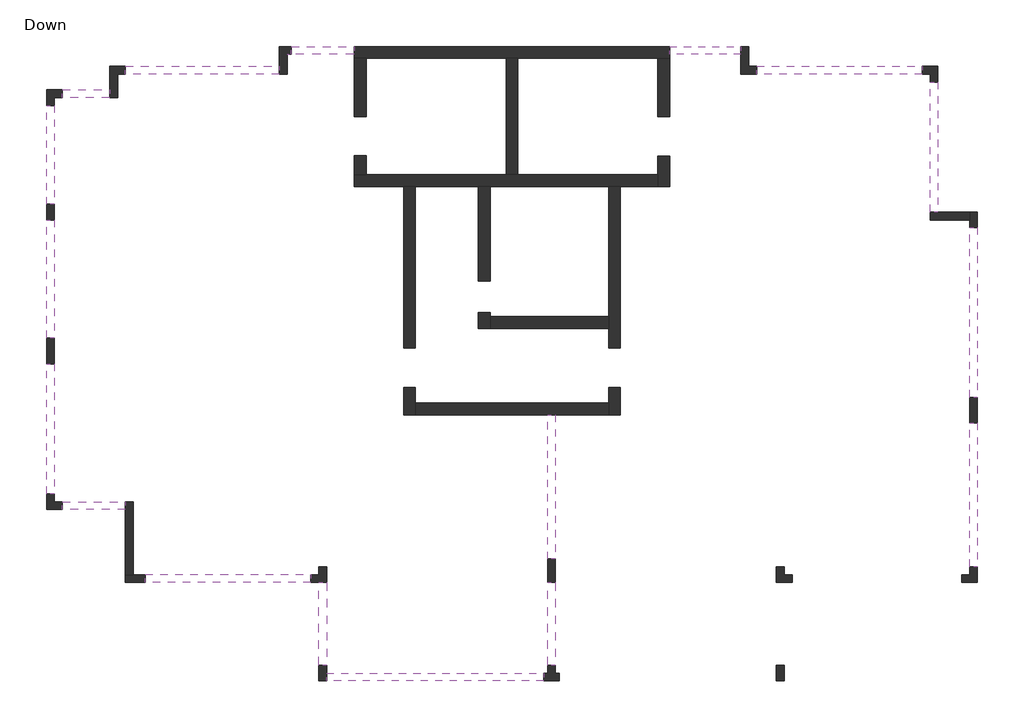
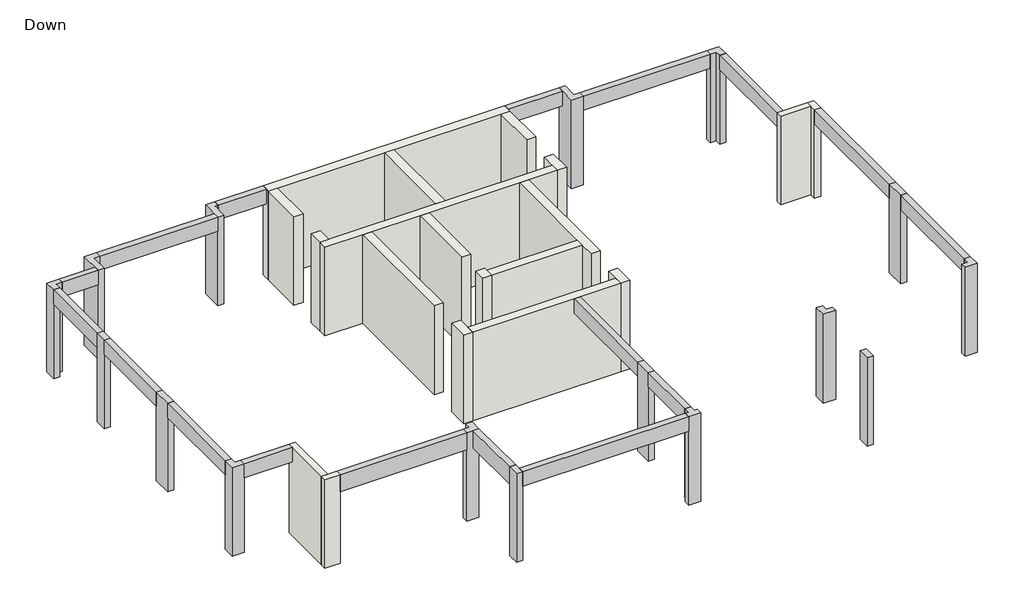
# One storey: 19 walls, 17 beams, 16 columns.
# Revit data of these elements (continued)
# Element 39 (IfcWall, "30") (continued)
#   SOFiSTiK_AMG_Scheduled = yes
#   SOFiSTiK_AMG_Adjusted = yes
#   Phase Created = New Construction
#   Base Constraint = Down
#   Top Constraint = Typical Floor
#   Materials on its faces: "Concrete"
# Element 40 (IfcWall, "30")
#   Comments = ""
#   Mark = "W7"
#   SOFiSTiK_EdgeZones = "W7"
#   SOFiSTiK_AMG_Comments = ""
#   Top Offset = 0 cm
#   Base Offset = 0 cm
#   wall height = 310 cm
#   SOFiSTiK_AMG_Scheduled = yes
#   SOFiSTiK_AMG_Adjusted = yes
#   Phase Created = New Construction
#   Base Constraint = Down
#   Top Constraint = Typical Floor
#   Materials on its faces: "Concrete"
# Element 41 (IfcWall, "30")
#   Comments = ""
#   Mark = "W8"
#   SOFiSTiK_EdgeZones = "W8"
#   SOFiSTiK_AMG_Comments = ""
#   Top Offset = 0 cm
#   Base Offset = 0 cm
#   wall height = 310 cm
#   SOFiSTiK_AMG_Scheduled = yes
#   SOFiSTiK_AMG_Adjusted = yes
#   Phase Created = New Construction
#   Base Constraint = Down
#   Top Constraint = Typical Floor
#   Materials on its faces: "Concrete"
# Element 42 (IfcWall, "30")
#   Comments = ""
#   Mark = "W9"
#   SOFiSTiK_EdgeZones = "W9"
#   SOFiSTiK_AMG_Comments = ""
#   Top Offset = 0 cm
#   Base Offset = 0 cm
#   wall height = 310 cm
#   SOFiSTiK_AMG_Scheduled = yes
#   SOFiSTiK_AMG_Adjusted = yes
#   Phase Created = New Construction
#   Base Constraint = Down
#   Top Constraint = Typical Floor
#   Materials on its faces: "Concrete"
# Element 43 (IfcWall, "30")
#   Comments = ""
#   Mark = "W10"
#   SOFiSTiK_EdgeZones = "W10"
#   SOFiSTiK_AMG_Comments = ""
#   Top Offset = 0 cm
#   Base Offset = 0 cm
#   wall height = 310 cm
#   SOFiSTiK_AMG_Scheduled = yes
#   SOFiSTiK_AMG_Adjusted = yes
#   Phase Created = New Construction
#   Base Constraint = Down
#   Top Constraint = Typical Floor
#   Materials on its faces: "Concrete"
# Element 44 (IfcWall, "30")
#   Comments = ""
#   Mark = "W11"
#   SOFiSTiK_EdgeZones = "W11"
#   SOFiSTiK_AMG_Comments = ""
#   Top Offset = 0 cm
#   Base Offset = 0 cm
#   wall height = 310 cm
#   SOFiSTiK_AMG_Scheduled = yes
#   SOFiSTiK_AMG_Adjusted = yes
#   Phase Created = New Construction
#   Base Constraint = Down
#   Top Constraint = Typical Floor
#   Materials on its faces: "Concrete"
# Element 45 (IfcWall, "30")
#   Comments = ""
#   Mark = "W12"
#   SOFiSTiK_EdgeZones = "W12"
#   SOFiSTiK_AMG_Comments = ""
#   Top Offset = 0 cm
#   Base Offset = 0 cm
#   wall height = 310 cm
#   SOFiSTiK_AMG_Scheduled = yes
#   SOFiSTiK_AMG_Adjusted = yes
#   Phase Created = New Construction
#   Base Constraint = Down
#   Top Constraint = Typical Floor
#   Materials on its faces: "Concrete"
# Element 46 (IfcWall, "30")
#   Comments = ""
#   Mark = "W13"
#   SOFiSTiK_EdgeZones = "W13"
#   SOFiSTiK_AMG_Comments = ""
#   Top Offset = 0 cm
#   Base Offset = 0 cm
#   wall height = 310 cm
#   SOFiSTiK_AMG_Scheduled = yes
#   SOFiSTiK_AMG_Adjusted = yes
#   Phase Created = New Construction
#   Base Constraint = Down
#   Top Constraint = Typical Floor
#   Materials on its faces: "Concrete"
# Element 47 (IfcWall, "30")
#   Comments = ""
#   Mark = "W14"
#   SOFiSTiK_EdgeZones = "W14"
#   SOFiSTiK_AMG_Comments = ""
#   Top Offset = 0 cm
#   Base Offset = 0 cm
#   wall height = 310 cm
#   SOFiSTiK_AMG_Scheduled = yes
#   SOFiSTiK_AMG_Adjusted = yes
#   Phase Created = New Construction
#   Base Constraint = Down
#   Top Constraint = Typical Floor
#   Materials on its faces: "Concrete"
# Element 48 (IfcWall, "30")
#   Comments = ""
#   Mark = "W15"
#   SOFiSTiK_EdgeZones = "W15"
#   SOFiSTiK_AMG_Comments = ""
#   Top Offset = 0 cm
#   Base Offset = 0 cm
#   wall height = 310 cm
#   SOFiSTiK_AMG_Scheduled = yes
#   SOFiSTiK_AMG_Adjusted = yes
#   Phase Created = New Construction
#   Base Constraint = Down
#   Top Constraint = Typical Floor
#   Materials on its faces: "Concrete"
# Element 49 (IfcWall, "30")
#   Comments = ""
#   Mark = "W16"
#   SOFiSTiK_EdgeZones = "W16"
#   SOFiSTiK_AMG_Comments = ""
#   Top Offset = 0 cm
#   Base Offset = 0 cm
#   wall height = 310 cm
#   SOFiSTiK_AMG_Scheduled = yes
#   SOFiSTiK_AMG_Adjusted = yes
#   Phase Created = New Construction
#   Base Constraint = Down
#   Top Constraint = Typical Floor
#   Materials on its faces: "Concrete"
# Element 50 (IfcWall, "30")
#   Comments = ""
#   Mark = "W17"
#   SOFiSTiK_EdgeZones = "W17"
#   SOFiSTiK_AMG_Comments = ""
#   Top Offset = 0 cm
#   Base Offset = 0 cm
#   wall height = 310 cm
#   SOFiSTiK_AMG_Scheduled = yes
#   SOFiSTiK_AMG_Adjusted = yes
#   Phase Created = New Construction
#   Base Constraint = Down
#   Top Constraint = Typical Floor
#   Materials on its faces: "Concrete"
# Element 51 (IfcWall, "30")
#   Comments = ""
#   Mark = "W18"
#   SOFiSTiK_EdgeZones = "W18"
#   SOFiSTiK_AMG_Comments = ""
#   Top Offset = 0 cm
#   Base Offset = 0 cm
#   wall height = 310 cm
#   SOFiSTiK_AMG_Scheduled = yes
#   SOFiSTiK_AMG_Adjusted = yes
#   Phase Created = New Construction
#   Base Constraint = Down
#   Top Constraint = Typical Floor
#   Materials on its faces: "Concrete"
# Element 52 (IfcWall, "30")
#   Comments = ""
#   Mark = "W19"
#   SOFiSTiK_EdgeZones = "W19"
#   SOFiSTiK_AMG_Comments = ""
#   Top Offset = 0 cm
#   Base Offset = 0 cm
#   wall height = 310 cm
#   SOFiSTiK_AMG_Scheduled = yes
#   SOFiSTiK_AMG_Adjusted = yes
#   Phase Created = New Construction
#   Base Constraint = Down
#   Top Constraint = Typical Floor
#   Materials on its faces: "Concrete"
# Materials
#   "Concrete": class "Concrete", colour RGB 192 192 192, transparency 0, Keynote = "01000", Description = "Cast-in-place concrete", Cost = 0
#   "Concrete, Cast-in-Place gray": class "Concrete", colour RGB 192 192 192, transparency 0, Description = "Cast-in-place concrete", Cost = 0
